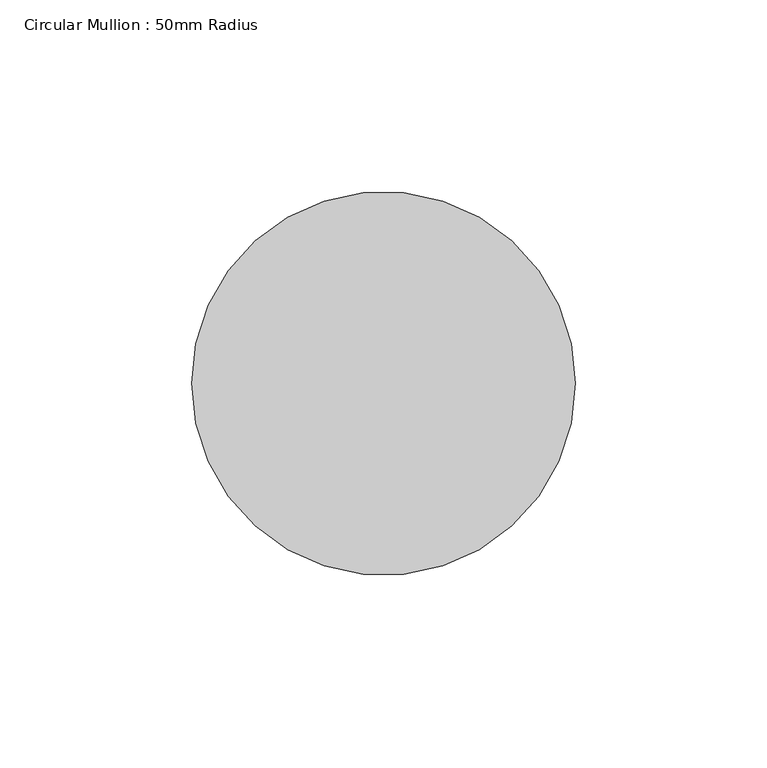
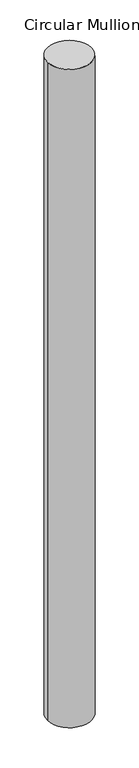
"""IFC4 building model written with IfcOpenShell, lengths in millimetres: member geometry, Circular Mullion : 50mm Radius."""

from ifc_helpers import new_model, si_unit, point, frame, origin, origin_2d, place, context, project, spatial, circle_curve, trimmed, segment, composite_curve, outline, extrude, source, transform, mapped, element, save


def circular_mullion_50mm_radius_4b55351b(model_context):
    return source(origin(), model_context, "Body", "SweptSolid", [
        extrude(outline(composite_curve([segment(trimmed(circle_curve(origin_2d(), 50.0), [point((50.0, 0.0))], [point((-50.0, 0.0))], False, "CARTESIAN"), True, "CONTINUOUS"), segment(trimmed(circle_curve(origin_2d(), 50.0), [point((-50.0, 0.0))], [point((50.0, 0.0))], False, "CARTESIAN"), True, "CONTINUOUS")], self_intersect=False)), frame((0.0, 0.0, -1579.1114208), z_axis=(0.0, 0.0, 1.0), x_axis=(1.0, 0.0, 0.0)), (0.0, 0.0, 1.0), 1579.1114208),
    ])


if __name__ == "__main__":
    model = new_model("IFC4")
    model_context = context("Model", 3, world=origin())
    ifc_project = project(units=[si_unit("LENGTHUNIT", "METRE", prefix="MILLI")], contexts=[model_context])
    site = spatial("IfcSite", under=ifc_project)
    building = spatial("IfcBuilding", under=site)
    placement = place(None, origin())
    circular_mullion_50mm_radius_shape = circular_mullion_50mm_radius_4b55351b(model_context)
    element("IfcMember", 1, ObjectType="Circular Mullion : 50mm Radius", at=placement, inside=building, context=model_context, shape_type="MappedRepresentation", body=[
        mapped(circular_mullion_50mm_radius_shape, transform((0.0, 0.0, 0.0), x_axis=(1.0, 0.0, 0.0), y_axis=(0.0, 1.0, 0.0), z_axis=(0.0, 0.0, 1.0))),
    ])
    save(model, "model.ifc")

# Revit data of these elements
# Type "Circular Mullion : 50mm Radius"
#   built-in parameter 1007350 = 0.164042 (stored number, unit not read)
# Element 1 (IfcMember, "Circular Mullion : 50mm Radius")
#   Materials on its faces: "Aluminium"
# Materials
#   "Aluminium": class "Metal", colour RGB 247 247 247, transparency 0, Description = "Aluminium 6061", Cost = 0
